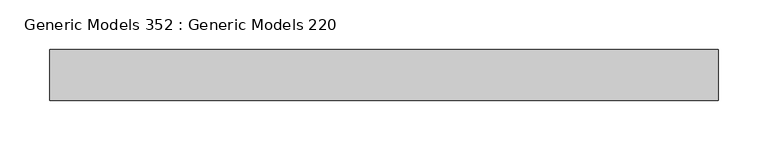
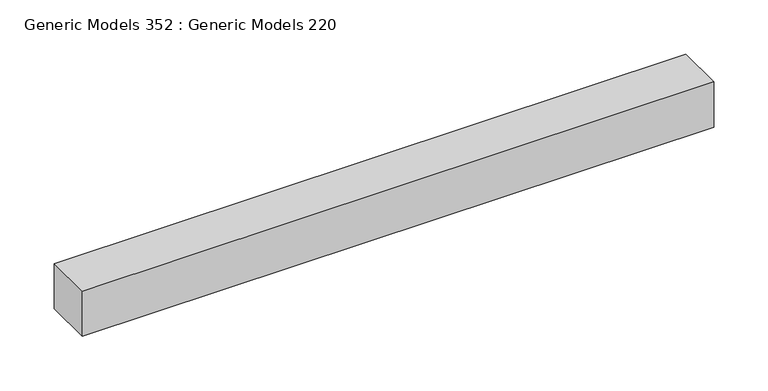
"""IFC4 building model written with IfcOpenShell, lengths in millimetres: proxy geometry, Generic Models 352 : Generic Models 220."""

from ifc_helpers import new_model, si_unit, frame, origin, place, context, project, spatial, polyline, outline, extrude, source, transform, mapped, element, save


def generic_models_352_generic_models_220_ab8ad24d(model_context):
    return source(origin(), model_context, "Body", "SweptSolid", [
        extrude(outline(polyline([(-6356.5236296, -4572.5730338), (-7026.3424842, -4572.5730338), (-7026.3424842, -4521.7730338), (-6356.5236296, -4521.7730338), (-6356.5236296, -4572.5730338)])), frame((0.0, 0.0, 129044.446), z_axis=(0.0, 0.0, 1.0), x_axis=(1.0, 0.0, 0.0)), (0.0, 0.0, 1.0), 50.8),
    ])


if __name__ == "__main__":
    model = new_model("IFC4")
    model_context = context("Model", 3, world=origin())
    ifc_project = project(units=[si_unit("LENGTHUNIT", "METRE", prefix="MILLI")], contexts=[model_context])
    site = spatial("IfcSite", under=ifc_project)
    building = spatial("IfcBuilding", under=site)
    placement = place(None, origin())
    generic_models_352_generic_models_220_shape = generic_models_352_generic_models_220_ab8ad24d(model_context)
    element("IfcBuildingElementProxy", 1, Name="Generic Models 352 : Generic Models 220", ObjectType="Generic Models 352 : Generic Models 220", at=placement, inside=building, context=model_context, shape_type="MappedRepresentation", body=[
        mapped(generic_models_352_generic_models_220_shape, transform((0.0, 0.0, 0.0), x_axis=(1.0, 0.0, 0.0), y_axis=(0.0, 1.0, 0.0), z_axis=(0.0, 0.0, 1.0))),
    ])
    save(model, "model.ifc")

# Revit data of these elements
# Element 1 (IfcBuildingElementProxy, "Generic Models 352 : Generic Models 220")
#   Materials on its faces: "_STRUCTURAL STEEL (SEE STRUCT. DWGS)"
# Materials
#   "_STRUCTURAL STEEL (SEE STRUCT. DWGS)": class "Metal", colour RGB 199 199 199, transparency 0, Description = "Structural steel 50ksi", Cost = 0
